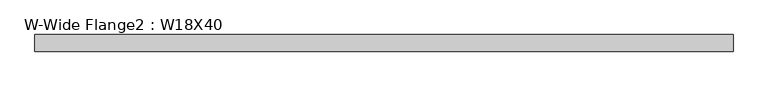
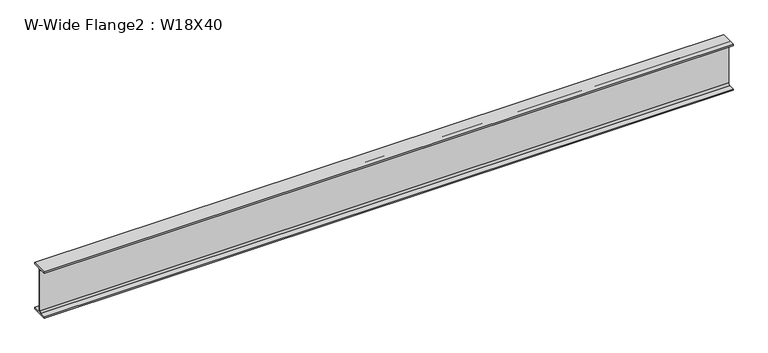
"""IFC4 building model written with IfcOpenShell, lengths in millimetres: beam geometry, W-Wide Flange2 : W18X40."""

from ifc_helpers import new_model, si_unit, point, frame, frame_2d, origin, place, context, project, spatial, polyline, circle_curve, trimmed, segment, composite_curve, outline, extrude, source, transform, mapped, element, save


def w_wide_flange2_w18x40_1ff26780(model_context):
    return source(origin(), model_context, "Body", "SweptSolid", [
        extrude(outline(composite_curve([segment(polyline([(76.454, -213.995), (76.454, -227.33), (-76.454, -227.33), (-76.454, -213.995), (-20.828, -213.995)]), True, "CONTINUOUS"), segment(trimmed(circle_curve(frame_2d((-20.828, -197.1675)), 16.8275), [point((-20.828, -213.995))], [point((-4.0005, -197.1675))], True, "CARTESIAN"), True, "CONTINUOUS"), segment(polyline([(-4.0005, -197.1675), (-4.0005, 197.1675)]), True, "CONTINUOUS"), segment(trimmed(circle_curve(frame_2d((-20.828, 197.1675)), 16.8275), [point((-4.0005, 197.1675))], [point((-20.828, 213.995))], True, "CARTESIAN"), True, "CONTINUOUS"), segment(polyline([(-20.828, 213.995), (-76.454, 213.995), (-76.454, 227.33), (76.454, 227.33), (76.454, 213.995), (20.828, 213.995)]), True, "CONTINUOUS"), segment(trimmed(circle_curve(frame_2d((20.828, 197.1675)), 16.8275), [point((20.828, 213.995))], [point((4.0005, 197.1675))], True, "CARTESIAN"), True, "CONTINUOUS"), segment(polyline([(4.0005, 197.1675), (4.0005, -197.1675)]), True, "CONTINUOUS"), segment(trimmed(circle_curve(frame_2d((20.828, -197.1675)), 16.8275), [point((4.0005, -197.1675))], [point((20.828, -213.995))], True, "CARTESIAN"), True, "CONTINUOUS"), segment(polyline([(20.828, -213.995), (76.454, -213.995)]), True, "CONTINUOUS")], self_intersect=False)), frame((-3206.353125, 0.0, 0.0), z_axis=(1.0, 0.0, 0.0), x_axis=(0.0, 1.0, 0.0)), (0.0, 0.0, 1.0), 6417.865625),
    ])


if __name__ == "__main__":
    model = new_model("IFC4")
    model_context = context("Model", 3, world=origin())
    ifc_project = project(units=[si_unit("LENGTHUNIT", "METRE", prefix="MILLI")], contexts=[model_context])
    site = spatial("IfcSite", under=ifc_project)
    building = spatial("IfcBuilding", under=site)
    placement = place(None, origin())
    w_wide_flange2_w18x40_shape = w_wide_flange2_w18x40_1ff26780(model_context)
    element("IfcBeam", 1, ObjectType="W-Wide Flange2 : W18X40", at=placement, inside=building, context=model_context, shape_type="MappedRepresentation", body=[
        mapped(w_wide_flange2_w18x40_shape, transform((0.0, 0.0, 0.0), x_axis=(1.0, 0.0, 0.0), y_axis=(0.0, 1.0, 0.0), z_axis=(0.0, 0.0, 1.0))),
    ])
    save(model, "model.ifc")

# Revit data of these elements
# Project information
#   Organization Name = "G3B Press"
#   Organization Description = "Paul F. Aubin Cosulting Services, Inc."
#   Building Name = "Revit Essentials for Architecture"
#   Author = "Paul F. Aubin"
#   Author Website = "https://www.paulaubin.com"
#   Copyright = "Copyright © 2020 Paul F Aubin, all rights reserved"
#   Project Issue Date = "8/1/2020"
#   Project Status = "Design Development"
#   Client Name = "Links Folder Version 1"
#   Project Address = "123 State ST\nSuite 301\nChicago, IL 60606"
#   Project Name = "Commercial-Structure"
#   Project Number = "2020.04S"
# Type "W-Wide Flange2 : W18X40"
#   Assembly Code = "B10"
#   W = 40
#   Length [instance default] = 5' - 0"
#   bf = 0' - 6.02"
#   d = 1' - 5.9"
#   k = 0' - 1 3/16"
#   k2 = 0' - 0.6625"
#   tf = 0' - 0.525"
#   tw = 0' - 0.315"
#   A = 0.0819444 SF
#   Structural Material [instance default] = Steel ASTM A992
# Element 1 (IfcBeam, "W-Wide Flange2 : W18X40")
#   Materials on its faces: "Steel ASTM A992"
# Materials
#   "Steel ASTM A992": class "Metal", colour RGB 199 199 199, transparency 0, Description = "Structural steel 50ksi", Cost = 0
